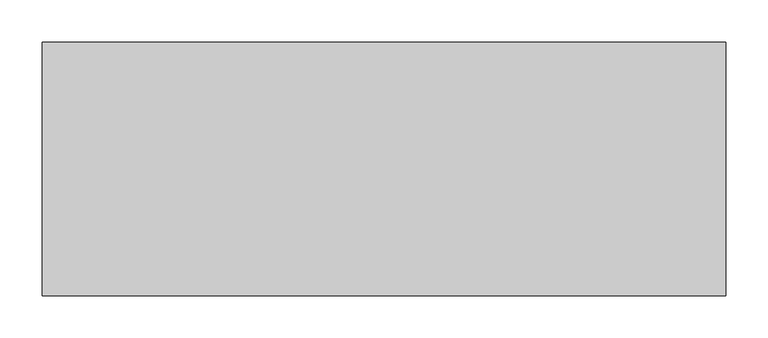
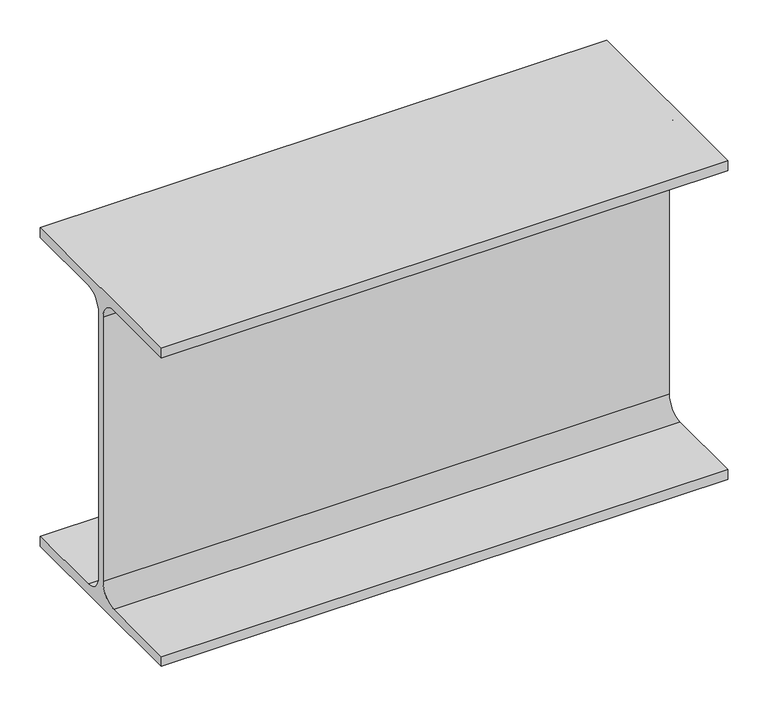
"""IFC4 building model written with IfcOpenShell, lengths in millimetres: beam geometry, 0912_Steel Framing_H-KSD3502 : H_SB_ASB_H-482x300x11x15."""

from ifc_helpers import new_model, si_unit, point, frame, frame_2d, origin, place, context, project, spatial, polyline, circle_curve, trimmed, segment, composite_curve, outline, extrude, source, transform, mapped, element, save


def beam_7ca781ba(model_context):
    return source(origin(), model_context, "Body", "SweptSolid", [
        extrude(outline(composite_curve([segment(polyline([(150.0, -226.0), (150.0, -241.0), (-150.0, -241.0), (-150.0, -226.0), (-31.5, -226.0)]), True, "CONTINUOUS"), segment(trimmed(circle_curve(frame_2d((-31.5, -200.0)), 26.0), [point((-31.5, -226.0))], [point((-5.5, -200.0))], True, "CARTESIAN"), True, "CONTINUOUS"), segment(polyline([(-5.5, -200.0), (-5.5, 200.0)]), True, "CONTINUOUS"), segment(trimmed(circle_curve(frame_2d((-31.5, 200.0)), 26.0), [point((-5.5, 200.0))], [point((-31.5, 226.0))], True, "CARTESIAN"), True, "CONTINUOUS"), segment(polyline([(-31.5, 226.0), (-150.0, 226.0), (-150.0, 241.0), (150.0, 241.0), (150.0, 226.0), (31.5, 226.0)]), True, "CONTINUOUS"), segment(trimmed(circle_curve(frame_2d((31.5, 200.0)), 26.0), [point((31.5, 226.0))], [point((5.5, 200.0))], True, "CARTESIAN"), True, "CONTINUOUS"), segment(polyline([(5.5, 200.0), (5.5, -200.0)]), True, "CONTINUOUS"), segment(trimmed(circle_curve(frame_2d((31.5, -200.0)), 26.0), [point((5.5, -200.0))], [point((31.5, -226.0))], True, "CARTESIAN"), True, "CONTINUOUS"), segment(polyline([(31.5, -226.0), (150.0, -226.0)]), True, "CONTINUOUS")], self_intersect=False)), frame((-404.8, 0.0, 0.0), z_axis=(1.0, 0.0, 0.0), x_axis=(0.0, 1.0, 0.0)), (0.0, 0.0, 1.0), 809.6),
    ])


if __name__ == "__main__":
    model = new_model("IFC4")
    model_context = context("Model", 3, world=origin())
    ifc_project = project(units=[si_unit("LENGTHUNIT", "METRE", prefix="MILLI")], contexts=[model_context])
    site = spatial("IfcSite", under=ifc_project)
    building = spatial("IfcBuilding", under=site)
    placement = place(None, origin())
    beam_shape = beam_7ca781ba(model_context)
    element("IfcBeam", 1, ObjectType="0912_Steel Framing_H-KSD3502 : H_SB_ASB_H-482x300x11x15", at=placement, inside=building, context=model_context, shape_type="MappedRepresentation", body=[
        mapped(beam_shape, transform((0.0, 0.0, 0.0), x_axis=(1.0, 0.0, 0.0), y_axis=(0.0, 1.0, 0.0), z_axis=(0.0, 0.0, 1.0))),
    ])
    save(model, "model.ifc")

# Revit data of these elements
# Type "0912_Steel Framing_H-KSD3502 : H_SB_ASB_H-482x300x11x15"
#   H_WM Code_1 = "S01AA001-00001 | Main Steel Structure Fabrication Work | Shelter/Building | Heavy Steel - Standard (Weight≥90KG/M) | Material: (   )"
#   H_WM Code_2 = "S03AA027-00001 | Main Steel Structure Erection Work | Shelter/Building | Heavy Steel (Weight≥90KG/M) | Material: (   )"
#   H_WM Code_3 = "S01AA010-00001 | Main Steel Structure Fabrication Work | Shelter/Building | Steel Painting/Coating | for Non-Fireproofed Steel Surface, Surface Preparation, Primer, Second & Final Coat | Material: (   )"
#   H_Q'ty Cal Type Tag = "SB-Q2"
#   Width = 30.0 cm
#   Web Thickness = 1.1 cm
#   Web Fillet = 2.6 cm
#   Warping Constant = 3680000.0 cm⁶
#   W = 0
#   Torsional Moment of Inertia = 88.2192 cm⁴
#   Section Area = 145.5 cm²
#   Plastic Modulus weak axis = 695.0 cm³
#   Plastic Modulus strong axis = 2790.0 cm³
#   Perimeter = 2.10 m²/m
#   Nominal Weight = 114.00 kgf/m
#   Moment of Inertia weak axis = 6760.00 cm⁴
#   Moment of Inertia strong axis = 60400.00 cm⁴
#   Height = 48.2 cm
#   Flange Thickness = 1.5 cm
#   Elastic Modulus weak axis = 451.0 cm³
#   Elastic Modulus strong axis = 2500.0 cm³
#   Centroid Vertical = 24.1 cm
#   Centroid Horizontal = 15.0 cm
#   Ix = 604000000
#   Length [instance default] = 1.5240 m
#   Zx = 2790000
#   b = 0.3000 m
#   h = 0.4820 m
#   r = 0.0260 m
#   s = 0.0110 m
#   t = 0.0150 m
#   A = 0.01455 m²
#   Structural Material [instance default] = Steel, 45-345
#   Assembly Code = ""
# Element 1 (IfcBeam, "0912_Steel Framing_H-KSD3502 : H_SB_ASB_H-482x300x11x15")
#   Structural Material = none
# Materials
#   "Steel, 45-345": class "Metal", colour RGB 189 187 185, transparency 0, Description = "Steel 345 MPa", Cost = 0
